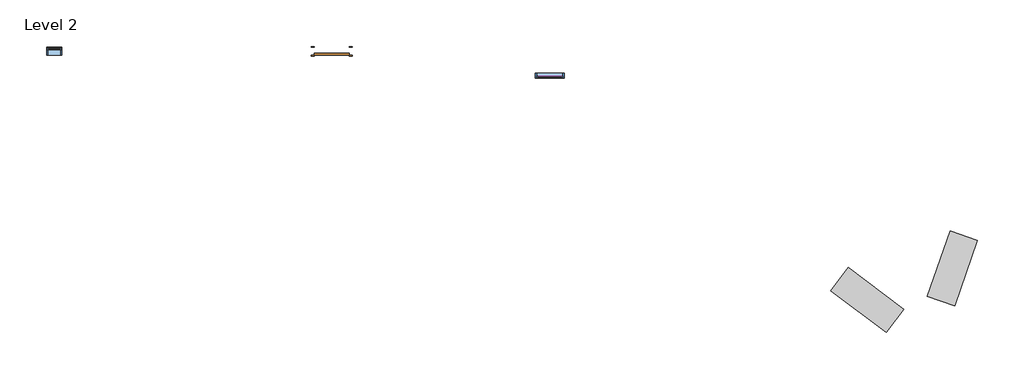
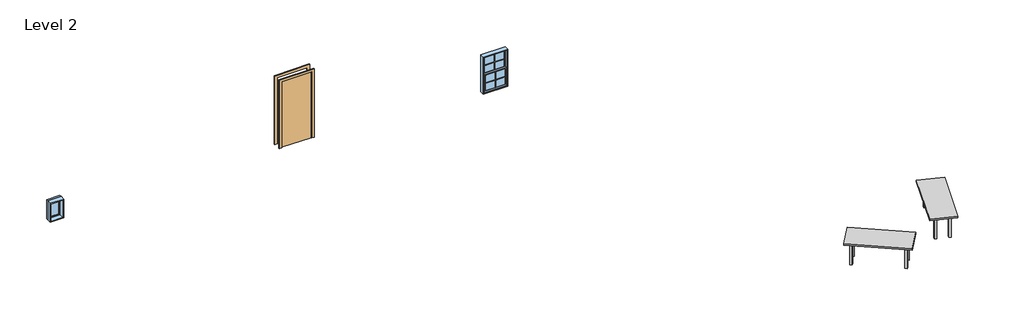
# One storey: 2 furniture elements, 2 proxies, 2 windows, 1 door.
"""IFC4 building model written with IfcOpenShell, lengths in millimetres."""

import ifcopenshell
import ifcopenshell.guid

model = None  # the IFC model being written
_history = None  # IfcOwnerHistory: only IFC2X3 demands one
_inside = {}  # id of a spatial element -> (the spatial element, [elements in it])
_under = {}  # id of a project, library or spatial element -> (it, [spatial elements below it])
_declared = {}  # id of a project -> (the project, [libraries it declares])
_typed = {}  # id of a type object -> (the type object, [elements of that type])
_made_of = {}  # id of a material, layer set ... -> (it, [elements and type objects made of it])


def new_model(schema):
    """Start an empty IFC model of exactly this schema.

    Asked for "IFC4X3", IfcOpenShell would pick the latest addendum, in which some entities
    have other attributes; the version numbers below select the first issue.
    IFC2X3 requires an IfcOwnerHistory on every rooted entity: one is made here for all.
    """
    global model, _history
    if schema == "IFC4X3":
        model = ifcopenshell.file(schema_version=(4, 3, 0, 0))
    else:
        model = ifcopenshell.file(schema=schema)
    _inside.clear()
    _under.clear()
    _declared.clear()
    _typed.clear()
    _made_of.clear()
    _history = None
    if model.schema == "IFC2X3":
        org = make("IfcOrganization", Name="unknown")
        user = make(
            "IfcPersonAndOrganization",
            ThePerson=make("IfcPerson", FamilyName="unknown"),
            TheOrganization=org,
        )
        app = make(
            "IfcApplication",
            ApplicationDeveloper=org,
            Version="unknown",
            ApplicationFullName="unknown",
            ApplicationIdentifier="unknown",
        )
        _history = make(
            "IfcOwnerHistory",
            OwningUser=user,
            OwningApplication=app,
            ChangeAction="ADDED",
            CreationDate=0,
        )
    return model


def make(cls, **values):
    """One entity of the class cls with the attributes given. An attribute that is None is left unset."""
    return model.create_entity(
        cls, **{name: value for name, value in values.items() if value is not None}
    )


def rooted(cls, **values):
    """An entity with a GlobalId (a new one), such as an element, a storey or a relation."""
    return make(cls, GlobalId=ifcopenshell.guid.new(), OwnerHistory=_history, **values)


def si_unit(unit_type, name, prefix=None):
    """IfcSIUnit, for example si_unit("LENGTHUNIT", "METRE", prefix="MILLI")."""
    return make("IfcSIUnit", UnitType=unit_type, Prefix=prefix, Name=name)


def assignment(units):
    """IfcUnitAssignment: the units of a project."""
    return None if units is None else make("IfcUnitAssignment", Units=units)


def point(xyz):
    """IfcCartesianPoint."""
    return None if xyz is None else make("IfcCartesianPoint", Coordinates=xyz)


def direction(xyz):
    """IfcDirection."""
    return None if xyz is None else make("IfcDirection", DirectionRatios=xyz)


def frame(location, z_axis=None, x_axis=None):
    """IfcAxis2Placement3D, a coordinate frame: its origin and axes. An axis left out is left unset."""
    return make(
        "IfcAxis2Placement3D",
        Location=point(location),
        Axis=direction(z_axis),
        RefDirection=direction(x_axis),
    )


def origin():
    """The frame at (0, 0, 0) with its axes left unset."""
    return frame((0.0, 0.0, 0.0))


def origin_with_axes():
    """The frame at (0, 0, 0) with the z axis (0, 0, 1) and the x axis (1, 0, 0) written out."""
    return frame((0.0, 0.0, 0.0), z_axis=(0.0, 0.0, 1.0), x_axis=(1.0, 0.0, 0.0))


def place(relative_to, where):
    """IfcLocalPlacement: puts the frame where relative to a parent placement (None: the world)."""
    return make(
        "IfcLocalPlacement", PlacementRelTo=relative_to, RelativePlacement=where
    )


def context(
    kind, dimensions, precision=None, world=None, true_north=None, identifier=None
):
    """IfcGeometricRepresentationContext, for example the 3D "Model" context."""
    return make(
        "IfcGeometricRepresentationContext",
        ContextIdentifier=identifier,
        ContextType=kind,
        CoordinateSpaceDimension=dimensions,
        Precision=precision,
        WorldCoordinateSystem=world,
        TrueNorth=true_north,
    )


def project(units=None, contexts=None):
    """IfcProject with its units and contexts."""
    return rooted(
        "IfcProject",
        Name="project",
        RepresentationContexts=contexts,
        UnitsInContext=assignment(units),
    )


def spatial(cls, under=None, at=None, **own):
    """A site, building, storey or space (cls), placed at a placement, below another one or the project."""
    s = rooted(cls, ObjectPlacement=at, **own)
    if under is not None:
        _under.setdefault(under.id(), (under, []))[1].append(s)
    return s


def polyline(points):
    """IfcPolyline through the points."""
    return make("IfcPolyline", Points=[point(p) for p in points])


def outline(outer, holes=None, kind="AREA"):
    """IfcArbitraryClosedProfileDef: a profile drawn as a closed curve; with holes, ...WithVoids."""
    if holes is None:
        return make("IfcArbitraryClosedProfileDef", ProfileType=kind, OuterCurve=outer)
    return make(
        "IfcArbitraryProfileDefWithVoids",
        ProfileType=kind,
        OuterCurve=outer,
        InnerCurves=holes,
    )


def extrude(swept, where, along, depth):
    """IfcExtrudedAreaSolid: the profile swept, set in the frame where, extruded along a direction by depth."""
    return make(
        "IfcExtrudedAreaSolid",
        SweptArea=swept,
        Position=where,
        ExtrudedDirection=direction(along),
        Depth=depth,
    )


def shape(context_of_items, identifier, shape_type, items):
    """IfcShapeRepresentation: the items that make up one representation, for example the "Body"."""
    return make(
        "IfcShapeRepresentation",
        ContextOfItems=context_of_items,
        RepresentationIdentifier=identifier,
        RepresentationType=shape_type,
        Items=items,
    )


def source(mapping_origin, context_of_items, identifier, shape_type, items):
    """IfcRepresentationMap: a shape defined once, which mapped items show again and again."""
    return make(
        "IfcRepresentationMap",
        MappingOrigin=mapping_origin,
        MappedRepresentation=shape(context_of_items, identifier, shape_type, items),
    )


def transform(
    local_origin,
    x_axis=None,
    y_axis=None,
    z_axis=None,
    scale=None,
    scale2=None,
    scale3=None,
    uniform=True,
):
    """IfcCartesianTransformationOperator3D, or its non-uniform kind. x_axis, y_axis, z_axis: its Axis1, 2, 3."""
    if uniform:
        return make(
            "IfcCartesianTransformationOperator3D",
            Axis1=direction(x_axis),
            Axis2=direction(y_axis),
            LocalOrigin=point(local_origin),
            Scale=scale,
            Axis3=direction(z_axis),
        )
    return make(
        "IfcCartesianTransformationOperator3DnonUniform",
        Axis1=direction(x_axis),
        Axis2=direction(y_axis),
        LocalOrigin=point(local_origin),
        Scale=scale,
        Axis3=direction(z_axis),
        Scale2=scale2,
        Scale3=scale3,
    )


def mapped(mapping_source, mapping_target):
    """IfcMappedItem: shows the shape of a source again, moved by a transform."""
    return make(
        "IfcMappedItem", MappingSource=mapping_source, MappingTarget=mapping_target
    )


def made_of(thing, what):
    """Note that an element or type object is made of a material, layer set ...; save() writes the relation."""
    if what is not None:
        _made_of.setdefault(what.id(), (what, []))[1].append(thing)
    return thing


def element(
    cls,
    number,
    at=None,
    inside=None,
    cuts=None,
    type_object=None,
    material=None,
    context=None,
    identifier="Body",
    shape_type=None,
    held_by="IfcProductDefinitionShape",
    body=None,
    shapes=None,
    **own,
):
    """One element of the class cls, such as IfcWall. Its Tag is "e" and its number.

    at: its placement. inside: the storey or other place that contains it. cuts: it is an
    opening in that element (IfcRelVoidsElement). A single representation is given by context,
    identifier, shape_type and body (its items); several are given by shapes. held_by: the class
    of the entity that holds the representations. save() writes the other relations.
    """
    e = rooted(cls, Tag="e%d" % number, ObjectPlacement=at, **own)
    if body is not None:
        shapes = [shape(context, identifier, shape_type, body)]
    if shapes is not None:
        e.Representation = make(held_by, Representations=shapes)
    if inside is not None:
        _inside.setdefault(inside.id(), (inside, []))[1].append(e)
    if cuts is not None:
        rooted(
            "IfcRelVoidsElement", RelatingBuildingElement=cuts, RelatedOpeningElement=e
        )
    if type_object is not None:
        _typed.setdefault(type_object.id(), (type_object, []))[1].append(e)
    return made_of(e, material)


def aggregate(whole, parts):
    """IfcRelAggregates: a whole, such as a stair, and the parts it consists of."""
    return rooted("IfcRelAggregates", RelatingObject=whole, RelatedObjects=parts)


def save(model, path):
    """Write the relations noted so far, then the file.

    IfcRelAggregates (storeys below a building ...), IfcRelContainedInSpatialStructure (elements
    in a storey), IfcRelDefinesByType, IfcRelAssociatesMaterial and IfcRelDeclares: one each for
    every whole, place, type object, material and project.
    """
    for whole, parts in _under.values():
        aggregate(whole, parts)
    for where, things in _inside.values():
        rooted(
            "IfcRelContainedInSpatialStructure",
            RelatedElements=things,
            RelatingStructure=where,
        )
    for kind, things in _typed.values():
        rooted("IfcRelDefinesByType", RelatedObjects=things, RelatingType=kind)
    for what, things in _made_of.values():
        rooted("IfcRelAssociatesMaterial", RelatedObjects=things, RelatingMaterial=what)
    for by, libraries in _declared.values():
        rooted("IfcRelDeclares", RelatingContext=by, RelatedDefinitions=libraries)
    model.write(path)


def m_muntin_pattern_2x2_m_muntin_pattern_2x2_aaec3afb(model_context):
    return source(origin(), model_context, "Body", "SweptSolid", [
        extrude(outline(polyline([(257.1375, -6.35), (257.1375, -298.8), (244.4375, -298.8), (244.4375, -6.35), (0.0, -6.35), (0.0, 6.35), (244.4375, 6.35), (244.4375, 298.8), (257.1375, 298.8), (257.1375, 6.35), (501.575, 6.35), (501.575, -6.35), (257.1375, -6.35)])), frame((0.0, 9.525, 0.0), z_axis=(0.0, 1.0, 0.0), x_axis=(0.0, 0.0, 1.0)), (0.0, 0.0, 1.0), 12.7),
        extrude(outline(polyline([(257.1375, -6.35), (257.1375, -298.8), (244.4375, -298.8), (244.4375, -6.35), (0.0, -6.35), (0.0, 6.35), (244.4375, 6.35), (244.4375, 298.8), (257.1375, 298.8), (257.1375, 6.35), (501.575, 6.35), (501.575, -6.35), (257.1375, -6.35)])), frame((0.0, -22.225, 0.0), z_axis=(0.0, 1.0, 0.0), x_axis=(0.0, 0.0, 1.0)), (0.0, 0.0, 1.0), 12.7),
    ])


def m_single_flush_0915_x_2134mm_6a9e8738(model_context):
    return source(origin(), model_context, "Body", "SweptSolid", [
        extrude(outline(polyline([(2210.0, -533.5), (0.0, -533.5), (0.0, -457.5), (2134.0, -457.5), (2134.0, 457.5), (0.0, 457.5), (0.0, 533.5), (2210.0, 533.5), (2210.0, -533.5)])), frame((0.0, 100.0, 0.0), z_axis=(0.0, 1.0, 0.0), x_axis=(0.0, 0.0, 1.0)), (0.0, 0.0, 1.0), 25.0),
        extrude(outline(polyline([(2210.0, 533.5), (2210.0, -533.5), (0.0, -533.5), (0.0, -457.5), (2134.0, -457.5), (2134.0, 457.5), (0.0, 457.5), (0.0, 533.5), (2210.0, 533.5)])), frame((0.0, -125.0, 0.0), z_axis=(0.0, 1.0, 0.0), x_axis=(0.0, 0.0, 1.0)), (0.0, 0.0, 1.0), 25.0),
        extrude(outline(polyline([(457.5, 49.0), (-457.5, 49.0), (-457.5, 100.0), (457.5, 100.0), (457.5, 49.0)])), origin_with_axes(), (0.0, 0.0, 1.0), 2134.0),
    ])


def m_table_rectangular_1830_x_0762mm_a0b3b7a0(model_context):
    return source(origin(), model_context, "Body", "SweptSolid", [
        extrude(outline(polyline([(699.1, 190.5), (699.1, 165.1), (-699.1, 165.1), (-699.1, 190.5), (699.1, 190.5)])), frame((0.0, 0.0, 609.6), z_axis=(0.0, 0.0, 1.0), x_axis=(1.0, 0.0, 0.0)), (0.0, 0.0, 1.0), 101.6),
        extrude(outline(polyline([(699.1, -190.5), (-699.1, -190.5), (-699.1, -165.1), (699.1, -165.1), (699.1, -190.5)])), frame((0.0, 0.0, 609.6), z_axis=(0.0, 0.0, 1.0), x_axis=(1.0, 0.0, 0.0)), (0.0, 0.0, 1.0), 101.6),
        extrude(outline(polyline([(-711.8, -165.1), (-737.2, -165.1), (-737.2, 165.1), (-711.8, 165.1), (-711.8, -165.1)])), frame((0.0, 0.0, 609.6), z_axis=(0.0, 0.0, 1.0), x_axis=(1.0, 0.0, 0.0)), (0.0, 0.0, 1.0), 101.6),
        extrude(outline(polyline([(711.8, -165.1), (711.8, 165.1), (737.2, 165.1), (737.2, -165.1), (711.8, -165.1)])), frame((0.0, 0.0, 609.6), z_axis=(0.0, 0.0, 1.0), x_axis=(1.0, 0.0, 0.0)), (0.0, 0.0, 1.0), 101.6),
        extrude(outline(polyline([(915.0, 381.0), (915.0, -381.0), (-915.0, -381.0), (-915.0, 381.0), (915.0, 381.0)])), frame((0.0, 0.0, 711.2), z_axis=(0.0, 0.0, 1.0), x_axis=(1.0, 0.0, 0.0)), (0.0, 0.0, 1.0), 50.8),
        extrude(outline(polyline([(-699.1, 228.6), (-699.1, 165.1), (-762.6, 165.1), (-762.6, 228.6), (-699.1, 228.6)])), origin_with_axes(), (0.0, 0.0, 1.0), 711.2),
        extrude(outline(polyline([(699.1, 228.6), (762.6, 228.6), (762.6, 165.1), (699.1, 165.1), (699.1, 228.6)])), origin_with_axes(), (0.0, 0.0, 1.0), 711.2),
        extrude(outline(polyline([(-699.1, -228.6), (-762.6, -228.6), (-762.6, -165.1), (-699.1, -165.1), (-699.1, -228.6)])), origin_with_axes(), (0.0, 0.0, 1.0), 711.2),
        extrude(outline(polyline([(699.1, -228.6), (699.1, -165.1), (762.6, -165.1), (762.6, -228.6), (699.1, -228.6)])), origin_with_axes(), (0.0, 0.0, 1.0), 711.2),
    ])


def m_fixed_0406_x_0610mm_8205b201(model_context):
    return source(origin(), model_context, "Body", "SweptSolid", [
        extrude(outline(polyline([(-140.0, 78.0), (140.0, 78.0), (140.0, 66.0), (-140.0, 66.0), (-140.0, 78.0)])), frame((0.0, 0.0, 978.0), z_axis=(0.0, 0.0, 1.0), x_axis=(1.0, 0.0, 0.0)), (0.0, 0.0, 1.0), 484.0),
        extrude(outline(polyline([(1506.0, -184.0), (934.0, -184.0), (934.0, 184.0), (1506.0, 184.0), (1506.0, -184.0)]), holes=[polyline([(1462.0, -140.0), (1462.0, 140.0), (978.0, 140.0), (978.0, -140.0), (1462.0, -140.0)])]), frame((0.0, 50.0, 0.0), z_axis=(0.0, 1.0, 0.0), x_axis=(0.0, 0.0, 1.0)), (0.0, 0.0, 1.0), 44.0),
        extrude(outline(polyline([(1525.0, -203.0), (915.0, -203.0), (915.0, 203.0), (1525.0, 203.0), (1525.0, -203.0)]), holes=[polyline([(1506.0, -184.0), (1506.0, 184.0), (934.0, 184.0), (934.0, -184.0), (1506.0, -184.0)])]), frame((0.0, 50.0, 0.0), z_axis=(0.0, 1.0, 0.0), x_axis=(0.0, 0.0, 1.0)), (0.0, 0.0, 1.0), 63.0),
        extrude(outline(polyline([(1525.0, -203.0), (915.0, -203.0), (915.0, 203.0), (1525.0, 203.0), (1525.0, -203.0)]), holes=[polyline([(1493.0, -171.0), (1493.0, 171.0), (947.0, 171.0), (947.0, -171.0), (1493.0, -171.0)])]), frame((0.0, -87.0, 0.0), z_axis=(0.0, 1.0, 0.0), x_axis=(0.0, 0.0, 1.0)), (0.0, 0.0, 1.0), 137.0),
    ])


def m_window_double_hung_750_x_1200mm_e7ea5f28(model_context):
    return source(origin(), model_context, "Body", "SweptSolid", [
        extrude(outline(polyline([(298.8, -669.85), (298.8, -676.2), (-298.8, -676.2), (-298.8, -669.85), (298.8, -669.85)])), frame((0.0, 0.0, 990.6), z_axis=(0.0, 0.0, 1.0), x_axis=(1.0, 0.0, 0.0)), (0.0, 0.0, 1.0), 501.575),
        extrude(outline(polyline([(-298.8, -682.55), (298.8, -682.55), (298.8, -688.9), (-298.8, -688.9), (-298.8, -682.55)])), frame((0.0, 0.0, 990.6), z_axis=(0.0, 0.0, 1.0), x_axis=(1.0, 0.0, 0.0)), (0.0, 0.0, 1.0), 501.575),
        extrude(outline(polyline([(298.8, -625.4), (298.8, -631.75), (-298.8, -631.75), (-298.8, -625.4), (298.8, -625.4)])), frame((0.0, 0.0, 1536.625), z_axis=(0.0, 0.0, 1.0), x_axis=(1.0, 0.0, 0.0)), (0.0, 0.0, 1.0), 501.575),
        extrude(outline(polyline([(-298.8, -638.1), (298.8, -638.1), (298.8, -644.45), (-298.8, -644.45), (-298.8, -638.1)])), frame((0.0, 0.0, 1536.625), z_axis=(0.0, 0.0, 1.0), x_axis=(1.0, 0.0, 0.0)), (0.0, 0.0, 1.0), 501.575),
        extrude(outline(polyline([(1536.625, -343.25), (946.15, -343.25), (946.15, 343.25), (1536.625, 343.25), (1536.625, -343.25)]), holes=[polyline([(1492.175, 298.8), (990.6, 298.8), (990.6, -298.8), (1492.175, -298.8), (1492.175, 298.8)])]), frame((0.0, -701.6, 0.0), z_axis=(0.0, 1.0, 0.0), x_axis=(0.0, 0.0, 1.0)), (0.0, 0.0, 1.0), 44.45),
        extrude(outline(polyline([(2082.65, -343.25), (1492.175, -343.25), (1492.175, 343.25), (2082.65, 343.25), (2082.65, -343.25)]), holes=[polyline([(2038.2, 298.8), (1536.625, 298.8), (1536.625, -298.8), (2038.2, -298.8), (2038.2, 298.8)])]), frame((0.0, -657.15, 0.0), z_axis=(0.0, 1.0, 0.0), x_axis=(0.0, 0.0, 1.0)), (0.0, 0.0, 1.0), 44.45),
        extrude(outline(polyline([(2114.4, -375.0), (914.4, -375.0), (914.4, 375.0), (2114.4, 375.0), (2114.4, -375.0)]), holes=[polyline([(2082.65, 343.25), (946.15, 343.25), (946.15, -343.25), (2082.65, -343.25), (2082.65, 343.25)])]), frame((0.0, -714.3, 0.0), z_axis=(0.0, 1.0, 0.0), x_axis=(0.0, 0.0, 1.0)), (0.0, 0.0, 1.0), 133.35),
    ])


model = new_model("IFC4")

# Units and contexts
model_context = context("Model", 3, world=origin())
ifc_project = project(units=[si_unit("LENGTHUNIT", "METRE", prefix="MILLI")], contexts=[model_context])

# Site, building, storey
site = spatial("IfcSite", under=ifc_project)
building = spatial("IfcBuilding", under=site)
storey = spatial("IfcBuildingStorey", under=building, Name="Level 2", Elevation=4000.0)

# Proxies
placement = place(None, origin())
m_muntin_pattern_2x2_m_muntin_pattern_2x2_shape = m_muntin_pattern_2x2_m_muntin_pattern_2x2_aaec3afb(model_context)
element("IfcBuildingElementProxy", 1, Name="M_Muntin Pattern_2x2 : M_Muntin Pattern_2x2", ObjectType="M_Muntin Pattern_2x2 : M_Muntin Pattern_2x2", at=placement, inside=storey, context=model_context, shape_type="MappedRepresentation", body=[
    mapped(m_muntin_pattern_2x2_m_muntin_pattern_2x2_shape, transform((-15264.9853759, 1399.5505832, 5536.625), x_axis=(1.0, 0.0, 0.0), y_axis=(0.0, 1.0, 0.0), z_axis=(0.0, 0.0, 1.0))),
])
element("IfcBuildingElementProxy", 2, Name="M_Muntin Pattern_2x2 : M_Muntin Pattern_2x2", ObjectType="M_Muntin Pattern_2x2 : M_Muntin Pattern_2x2", at=placement, inside=storey, context=model_context, shape_type="MappedRepresentation", body=[
    mapped(m_muntin_pattern_2x2_m_muntin_pattern_2x2_shape, transform((-15264.9853759, 1355.1005832, 4990.6), x_axis=(1.0, 0.0, 0.0), y_axis=(0.0, 1.0, 0.0), z_axis=(0.0, 0.0, 1.0))),
])

# Door
m_single_flush_0915_x_2134mm_shape = m_single_flush_0915_x_2134mm_6a9e8738(model_context)
element("IfcDoor", 3, ObjectType="M_Single-Flush : 0915 x 2134mm", at=placement, inside=storey, context=model_context, shape_type="MappedRepresentation", body=[
    mapped(m_single_flush_0915_x_2134mm_shape, transform((-20997.4853759, 2034.4755832, 4866.0), x_axis=(-1.0, 0.0, 0.0), y_axis=(0.0, -1.0, 0.0), z_axis=(0.0, 0.0, 1.0))),
])

# Furniture
m_table_rectangular_1830_x_0762mm_shape = m_table_rectangular_1830_x_0762mm_a0b3b7a0(model_context)
element("IfcFurniture", 4, ObjectType="M_Table-Rectangular : 1830 x 0762mm", at=placement, inside=storey, context=model_context, shape_type="MappedRepresentation", body=[
    mapped(m_table_rectangular_1830_x_0762mm_shape, transform((-4676.3852744, -3681.7142207, 0.0), x_axis=(-0.32556815445715137, -0.9455185755993186, 0.0), y_axis=(0.9455185755993186, -0.32556815445715137, 0.0), z_axis=(0.0, 0.0, 1.0))),
])
element("IfcFurniture", 5, ObjectType="M_Table-Rectangular : 1830 x 0762mm", at=placement, inside=storey, context=model_context, shape_type="MappedRepresentation", body=[
    mapped(m_table_rectangular_1830_x_0762mm_shape, transform((-6912.0232604, -4514.409007, 0.0), x_axis=(0.7986355100472892, -0.601815023152053, 0.0), y_axis=(0.601815023152053, 0.7986355100472892, 0.0), z_axis=(0.0, 0.0, 1.0))),
])

# Windows
m_fixed_0406_x_0610mm_shape = m_fixed_0406_x_0610mm_8205b201(model_context)
element("IfcWindow", 6, ObjectType="M_Fixed : 0406 x 0610mm", at=placement, inside=storey, context=model_context, shape_type="MappedRepresentation", body=[
    mapped(m_fixed_0406_x_0610mm_shape, transform((-28293.5284847, 2021.4755832, 4000.0), x_axis=(1.0, 0.0, 0.0), y_axis=(0.0, 1.0, 0.0), z_axis=(0.0, 0.0, 1.0))),
])
m_window_double_hung_750_x_1200mm_shape = m_window_double_hung_750_x_1200mm_e7ea5f28(model_context)
element("IfcWindow", 7, ObjectType="M_Window-Double-Hung : 750 x 1200mm", at=placement, inside=storey, context=model_context, shape_type="MappedRepresentation", body=[
    mapped(m_window_double_hung_750_x_1200mm_shape, transform((-15264.9853759, 2034.4755832, 4000.0), x_axis=(1.0, 0.0, 0.0), y_axis=(0.0, 1.0, 0.0), z_axis=(0.0, 0.0, 1.0))),
])

save(model, "model.ifc")

# Revit data of these elements
# Type "M_Muntin Pattern_2x2 : M_Muntin Pattern_2x2"
#   Width [instance default] = 1200 mm
#   Thickness = 12.7 mm
#   Height [instance default] = 1200 mm
#   Distance = 19.05 mm
#   Interior Material [instance default] = none
#   Exterior Material [instance default] = none
#   Default Elevation = 0
# Type "M_Single-Flush : 0915 x 2134mm"
#   Type Mark = "20"
#   Construction Type Id = "MDOOR"
#   Analytic Construction = "Metal"
#   Thickness = 51 mm
#   Thermal Resistance (R) = 0.270117 (m²·K)/W
#   Heat Transfer Coefficient (U) = 3.7021 W/(m²·K)
#   Height = 2134 mm
#   Trim Projection Ext = 25 mm
#   Trim Projection Int = 25 mm
#   Trim Width = 76 mm
#   Width = 915 mm
#   Define Thermal Properties by = 1
#   Define Thermal Properties by = 1
#   Door Material = Door - Panel
#   Frame Material = Door - Frame
#   Visual Light Transmittance = 0
#   Solar Heat Gain Coefficient = 0
#   Function = (empty or 0)
#   Wall Closure = (empty or 0)
# Type "M_Table-Rectangular : 1830 x 0762mm"
#   Height = 762 mm
#   Length = 1830 mm
#   Width = 762 mm
#   Base Material = Birch
#   Top Material = Birch
#   Default Elevation = 0
# Type "M_Fixed : 0406 x 0610mm"
#   Type Mark = "10"
#   Construction Type Id = "GSP4R"
#   Analytic Construction = "1/8 in Pilkington single glazing"
#   Visual Light Transmittance = 0.9
#   Thermal Resistance (R) = 0.271106 (m²·K)/W
#   Solar Heat Gain Coefficient = 0.78
#   Heat Transfer Coefficient (U) = 3.6886 W/(m²·K)
#   Height = 610 mm
#   Default Sill Height = 915 mm
#   Width = 406 mm
#   Window Inset = 19 mm
#   Define Thermal Properties by = 1
#   Define Thermal Properties by = 1
#   Frame Exterior Material = Sash
#   Frame Interior Material = Sash
#   Glass Pane Material = Glass
#   Sash = Sash
#   Wall Closure = (empty or 0)
# Type "M_Window-Double-Hung : 750 x 1200mm"
#   Type Mark = "22"
#   Fire Rating = "0.5h"
#   Construction Type Id = "DG-DR"
#   Assembly Code = "B2020100"
#   Analytic Construction = "Double glazing - domestic"
#   Wall Thickness [instance default] = 150 mm
#   Window Inset [instance default] = 0 mm
#   Visual Light Transmittance = 0.81
#   Thermal Resistance (R) = 0.319569 (m²·K)/W
#   Solar Heat Gain Coefficient = 0.76
#   Muntin Width = 597.6 mm
#   Muntin Height = 501.575 mm
#   Interior Wall Closure [instance default] = 35.7 mm
#   Rough Width = 765 mm
#   Rough Height = 1215 mm
#   Frame Extension [instance default] = 31.75 mm
#   Exterior Wall Closure [instance default] = 12.7 mm
#   Extension Jamb [instance default] = 35.7 mm
#   Heat Transfer Coefficient (U) = 3.12929 W/(m²·K)
#   Height = 1200 mm
#   Width = 750 mm
#   Define Thermal Properties by = 1
#   Top Muntin Visibility = yes
#   Indicator Visibility [instance default] = yes
#   Extension Jamb Visibility [instance default] = yes
#   Interior Trim Visibility [instance default] = yes
#   Exterior Trim Visibility [instance default] = yes
#   Define Thermal Properties by = 1
#   Bottom Muntin Visibility = yes
#   Muntin Pattern = M_Muntin Pattern_2x2 : M_Muntin Pattern_2x2
#   Interior Trim Material = Wood - Stained
#   Interior Trim = M_Trim-Window-Interior-Flat : Picture Frame
#   Exterior Trim Material = Clad - White
#   Exterior Trim = M_Trim-Window-Exterior-Flat : with Sill
#   Glass Panel Material = Glass
#   Exterior Frame Material = Clad - White
#   Interior Frame Material = Wood - Stained
#   Wall Closure = (empty or 0)
# Elements 1, 2 (IfcBuildingElementProxy, "M_Muntin Pattern_2x2 : M_Muntin Pattern_2x2")
#   Width = 597.6 mm
#   Height = 501.575 mm
#   Interior Material = Wood - Stained
#   Exterior Material = Clad - White
#   Phase Created = New Construction
#   Materials on its faces: "Clad - White", "Wood - Stained"
# Element 3 (IfcDoor, "M_Single-Flush : 0915 x 2134mm")
#   SpeckleObjectUpdateDescription = "location change"
#   SpeckleObjectTestNumber = 5
#   Phase Created = New Construction
#   Materials on its faces: "Door - Frame", "Door - Panel"
# Element 4 (IfcFurniture, "M_Table-Rectangular : 1830 x 0762mm")
#   SpeckleObjectUpdateDescription = "Hosted element rotation"
#   SpeckleObjectTestNumber = 10
#   Phase Created = New Construction
#   Materials on its faces: "Birch"
# Element 5 (IfcFurniture, "M_Table-Rectangular : 1830 x 0762mm")
#   SpeckleObjectUpdateDescription = "level change"
#   SpeckleObjectTestNumber = 11
#   Phase Created = New Construction
#   Materials on its faces: "Birch"
# Element 6 (IfcWindow, "M_Fixed : 0406 x 0610mm")
#   Mark = "1"
#   SpeckleObjectUpdateDescription = "level change"
#   SpeckleObjectTestNumber = 2
#   Phase Created = New Construction
#   Materials on its faces: "Sash", "Glass"
# Element 7 (IfcWindow, "M_Window-Double-Hung : 750 x 1200mm")
#   Mark = "4"
#   SpeckleObjectUpdateDescription = "None yet"
#   Window Inset = 700 mm
#   Interior Wall Closure = 60 mm
#   Frame Extension = 31.75 mm
#   Exterior Wall Closure = 50 mm
#   SpeckleObjectTestNumber = 7
#   Interior Trim Visibility = no
#   Indicator Visibility = no
#   Exterior Trim Visibility = no
#   Phase Created = New Construction
#   Materials on its faces: "Wood - Stained", "Glass", "Clad - White"
# Materials
#   "Door - Panel": class "Wood", colour RGB 210 159 95, transparency 0, Cost = 0
#   "Door - Frame": class "Miscellaneous", colour RGB 118 70 51, transparency 0, Cost = 0
#   "Birch": class "Wood", colour RGB 224 178 126, transparency 0, Description = "Betula Alleghaniensis", Cost = 0
#   "Sash": class "Wood", colour RGB 224 178 126, transparency 0, Cost = 0
#   "Glass": class "Glass", colour RGB 0 128 192, transparency 0.9, Description = "Soda Lime Glass", Cost = 0
#   "Wood - Stained": class "Wood", colour RGB 224 178 126, transparency 0, Cost = 0
#   "Clad - White": class "Wood", colour RGB 242 242 238, transparency 0, Cost = 0
